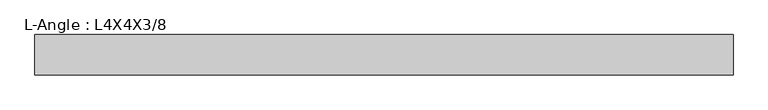
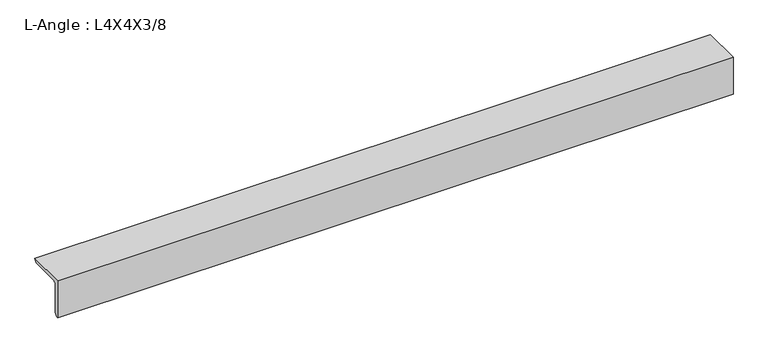
"""IFC4 building model written with IfcOpenShell, lengths in millimetres: beam geometry, L-Angle : L4X4X3/8."""

from ifc_helpers import new_model, si_unit, point, frame, frame_2d, origin, place, context, project, spatial, polyline, circle_curve, trimmed, segment, composite_curve, outline, extrude, source, transform, mapped, element, save


def l_angle_l4x4x3_8_db77c512(model_context):
    return source(origin(), model_context, "Body", "SweptSolid", [
        extrude(outline(composite_curve([segment(polyline([(-28.702, 28.702), (72.898, 28.702)]), True, "CONTINUOUS"), segment(trimmed(circle_curve(frame_2d((63.373, 28.702)), 9.525), [point((72.898, 28.702))], [point((63.373, 19.177))], False, "CARTESIAN"), True, "CONTINUOUS"), segment(polyline([(63.373, 19.177), (-9.652, 19.177)]), True, "CONTINUOUS"), segment(trimmed(circle_curve(frame_2d((-9.652, 9.652)), 9.525), [point((-9.652, 19.177))], [point((-19.177, 9.652))], True, "CARTESIAN"), True, "CONTINUOUS"), segment(polyline([(-19.177, 9.652), (-19.177, -63.373)]), True, "CONTINUOUS"), segment(trimmed(circle_curve(frame_2d((-28.702, -63.373)), 9.525), [point((-19.177, -63.373))], [point((-28.702, -72.898))], False, "CARTESIAN"), True, "CONTINUOUS"), segment(polyline([(-28.702, -72.898), (-28.702, 28.702)]), True, "CONTINUOUS")], self_intersect=False)), frame((-863.6, 0.0, 0.0), z_axis=(1.0, 0.0, 0.0), x_axis=(0.0, 1.0, 0.0)), (0.0, 0.0, 1.0), 1752.6),
    ])


if __name__ == "__main__":
    model = new_model("IFC4")
    model_context = context("Model", 3, world=origin())
    ifc_project = project(units=[si_unit("LENGTHUNIT", "METRE", prefix="MILLI")], contexts=[model_context])
    site = spatial("IfcSite", under=ifc_project)
    building = spatial("IfcBuilding", under=site)
    placement = place(None, origin())
    l_angle_l4x4x3_8_shape = l_angle_l4x4x3_8_db77c512(model_context)
    element("IfcBeam", 1, ObjectType="L-Angle : L4X4X3/8", at=placement, inside=building, context=model_context, shape_type="MappedRepresentation", body=[
        mapped(l_angle_l4x4x3_8_shape, transform((0.0, 0.0, 0.0), x_axis=(1.0, 0.0, 0.0), y_axis=(0.0, 1.0, 0.0), z_axis=(0.0, 0.0, 1.0))),
    ])
    save(model, "model.ifc")

# Revit data of these elements
# Type "L-Angle : L4X4X3/8"
#   Assembly Code = "B10"
#   k = 0' - 0 3/4"
#   W = 9.8
#   Length [instance default] = 5' - 0"
#   b = 0' - 4"
#   d = 0' - 4"
#   t = 0' - 0 3/8"
#   x = 0' - 1.13"
#   y = 0' - 1.13"
#   A = 0.0198611 SF
#   Structural Material [instance default] = Steel ASTM A36
# Element 1 (IfcBeam, "L-Angle : L4X4X3/8")
#   Materials on its faces: "Steel ASTM A36"
# Materials
#   "Steel ASTM A36": class "Metal", colour RGB 199 199 199, transparency 0, Description = "Structural steel, ASTM A36 Grade B, mill finish", Cost = 0
